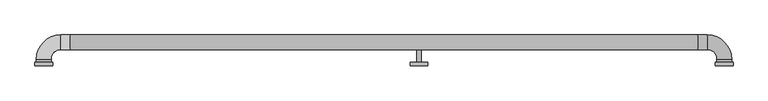
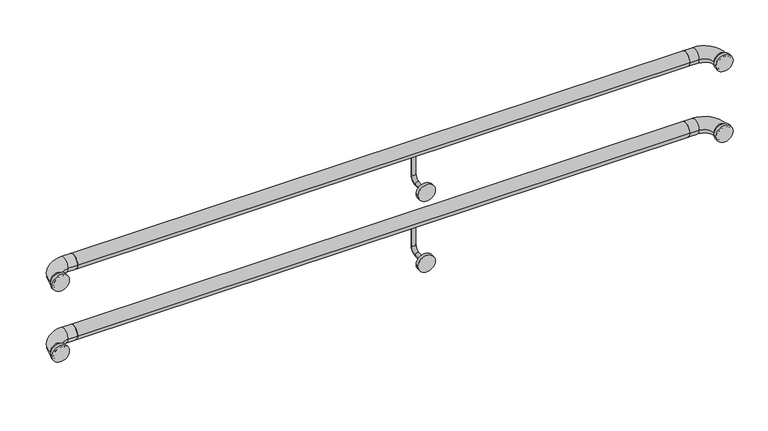
"""IFC4 building model written with IfcOpenShell, lengths in millimetres: railing geometry."""

from ifc_helpers import new_model, si_unit, point, frame, frame_2d, origin, place, context, project, spatial, circle_curve, ellipse_curve, trimmed, segment, composite_curve, outline, extrude, source, transform, mapped, element, save
from ifc_brep_helpers import plane_surface, cylinder_surface, revolved_surface, advanced_brep


def railing_3e29a62d(model_context):
    return source(origin(), model_context, "Body", "SolidModel", [
        extrude(outline(composite_curve([segment(trimmed(circle_curve(frame_2d((33728.1400611, 899.0)), 21.0), [point((33749.1400611, 899.0))], [point((33707.1400611, 899.0))], False, "CARTESIAN"), True, "CONTINUOUS"), segment(trimmed(circle_curve(frame_2d((33728.1400611, 899.0)), 21.0), [point((33707.1400611, 899.0))], [point((33749.1400611, 899.0))], False, "CARTESIAN"), True, "CONTINUOUS")], self_intersect=False)), frame((9766.6129185, 0.0, 0.0), z_axis=(1.0, 0.0, 0.0), x_axis=(0.0, 1.0, 0.0)), (0.0, 0.0, 1.0), 1800.0),
        extrude(outline(composite_curve([segment(trimmed(circle_curve(frame_2d((33728.1400611, 679.0)), 21.0), [point((33749.1400611, 679.0))], [point((33707.1400611, 679.0))], False, "CARTESIAN"), True, "CONTINUOUS"), segment(trimmed(circle_curve(frame_2d((33728.1400611, 679.0)), 21.0), [point((33707.1400611, 679.0))], [point((33749.1400611, 679.0))], False, "CARTESIAN"), True, "CONTINUOUS")], self_intersect=False)), frame((9766.6129185, 0.0, 0.0), z_axis=(1.0, 0.0, 0.0), x_axis=(0.0, 1.0, 0.0)), (0.0, 0.0, 1.0), 1800.0),
        extrude(outline(composite_curve([segment(trimmed(circle_curve(frame_2d((582.0, 10766.6129185)), 25.4), [point((582.0, 10792.0129185))], [point((582.0, 10741.2129185))], False, "CARTESIAN"), True, "CONTINUOUS"), segment(trimmed(circle_curve(frame_2d((582.0, 10766.6129185)), 25.4), [point((582.0, 10741.2129185))], [point((582.0, 10792.0129185))], False, "CARTESIAN"), True, "CONTINUOUS")], self_intersect=False)), frame((0.0, 33661.1900611, 0.0), z_axis=(0.0, 1.0, 0.0), x_axis=(0.0, 0.0, 1.0)), (0.0, 0.0, 1.0), 9.525),
        extrude(outline(composite_curve([segment(trimmed(circle_curve(frame_2d((802.0, 10766.6129185)), 25.4), [point((802.0, 10792.0129185))], [point((802.0, 10741.2129185))], False, "CARTESIAN"), True, "CONTINUOUS"), segment(trimmed(circle_curve(frame_2d((802.0, 10766.6129185)), 25.4), [point((802.0, 10741.2129185))], [point((802.0, 10792.0129185))], False, "CARTESIAN"), True, "CONTINUOUS")], self_intersect=False)), frame((0.0, 33661.1900611, 0.0), z_axis=(0.0, 1.0, 0.0), x_axis=(0.0, 0.0, 1.0)), (0.0, 0.0, 1.0), 9.525),
        advanced_brep(
        [(10760.2629185, 33728.1900611, 658.0), (10772.9629185, 33728.1900611, 658.0), (10760.2629185, 33728.1900611, 601.05), (10772.9629185, 33728.1900611, 601.05), (10772.9629185, 33709.1400611, 582.0), (10760.2629185, 33709.1400611, 582.0), (10760.2629185, 33670.7150611, 582.0), (10772.9629185, 33670.7150611, 582.0)],
        [
            (0, 1, circle_curve(frame((10766.6129185, 33728.1900611, 658.0), z_axis=(0.0, 0.0, 1.0), x_axis=(1.0, 0.0, 0.0)), 6.35)),
            (1, 0, circle_curve(frame((10766.6129185, 33728.1900611, 658.0), z_axis=(0.0, 0.0, 1.0), x_axis=(1.0, 0.0, 0.0)), 6.35)),
            (0, 2),
            (2, 3, circle_curve(frame((10766.6129185, 33728.1900611, 601.05), z_axis=(0.0, 0.0, 1.0), x_axis=(1.0, 0.0, 0.0)), 6.35)),
            (3, 1),
            (3, 2, circle_curve(frame((10766.6129185, 33728.1900611, 601.05), z_axis=(0.0, 0.0, 1.0), x_axis=(1.0, 0.0, 0.0)), 6.35)),
            (4, 3, circle_curve(frame((10772.9629185, 33709.1400611, 601.05), z_axis=(1.0, 0.0, 0.0), x_axis=(0.0, 1.0, 0.0)), 19.05)),
            (2, 5, circle_curve(frame((10760.2629185, 33709.1400611, 601.05), z_axis=(-1.0, 0.0, 0.0), x_axis=(0.0, 1.0, 0.0)), 19.05)),
            (5, 4, circle_curve(frame((10766.6129185, 33709.1400611, 582.0), z_axis=(0.0, 1.0, 0.0), x_axis=(1.0, 0.0, 0.0)), 6.35)),
            (4, 5, circle_curve(frame((10766.6129185, 33709.1400611, 582.0), z_axis=(0.0, 1.0, 0.0), x_axis=(1.0, 0.0, 0.0)), 6.35)),
            (6, 7, circle_curve(frame((10766.6129185, 33670.7150611, 582.0), z_axis=(0.0, -1.0, 0.0), x_axis=(1.0, 0.0, 0.0)), 6.35)),
            (7, 6, circle_curve(frame((10766.6129185, 33670.7150611, 582.0), z_axis=(0.0, -1.0, 0.0), x_axis=(1.0, 0.0, 0.0)), 6.35)),
            (5, 6),
            (7, 4),
        ],
        [
            plane_surface(frame((10772.9629185, 33728.1900611, 658.0), z_axis=(0.0, 0.0, 1.0), x_axis=(0.0, -1.0, 0.0))),
            cylinder_surface(frame((10766.6129185, 33728.1900611, 658.0), z_axis=(0.0, 0.0, 1.0), x_axis=(1.0, 0.0, 0.0)), 6.35),
            revolved_surface(trimmed(ellipse_curve(frame((10766.6129185, 33728.1900611, 601.05), z_axis=(0.0, 0.0, 1.0), x_axis=(1.0, 0.0, 0.0)), 6.35, 6.35), [point((10760.2629185, 33728.1900611, 601.05))], [point((10772.9629185, 33728.1900611, 601.05))], True, "CARTESIAN"), (10766.6129185, 33709.1400611, 601.05), (-1.0, 0.0, 0.0)),
            revolved_surface(trimmed(ellipse_curve(frame((10766.6129185, 33728.1900611, 601.05), z_axis=(0.0, 0.0, 1.0), x_axis=(1.0, 0.0, 0.0)), 6.35, 6.35), [point((10772.9629185, 33728.1900611, 601.05))], [point((10760.2629185, 33728.1900611, 601.05))], True, "CARTESIAN"), (10766.6129185, 33709.1400611, 601.05), (-1.0, 0.0, 0.0)),
            plane_surface(frame((10766.6129185, 33670.7150611, 575.65), z_axis=(0.0, -1.0, 0.0), x_axis=(1.0, 0.0, 0.0))),
            cylinder_surface(frame((10766.6129185, 33709.1400611, 582.0), z_axis=(0.0, 1.0, 0.0), x_axis=(1.0, 0.0, 0.0)), 6.35),
        ],
        [
            (0, [[1, 2]]),
            (1, [[-1, 3, 4, 5]]),
            (1, [[-2, -5, 6, -3]]),
            (2, [[7, -4, 8, 9]]),
            (3, [[-8, -6, -7, 10]]),
            (4, [[11, 12]]),
            (5, [[-9, 13, -12, 14]]),
            (5, [[-10, -14, -11, -13]]),
        ],
    ),
        advanced_brep(
        [(10760.2629185, 33728.1900611, 878.0), (10772.9629185, 33728.1900611, 878.0), (10760.2629185, 33728.1900611, 821.05), (10772.9629185, 33728.1900611, 821.05), (10772.9629185, 33709.1400611, 802.0), (10760.2629185, 33709.1400611, 802.0), (10760.2629185, 33670.7150611, 802.0), (10772.9629185, 33670.7150611, 802.0)],
        [
            (0, 1, circle_curve(frame((10766.6129185, 33728.1900611, 878.0), z_axis=(0.0, 0.0, 1.0), x_axis=(1.0, 0.0, 0.0)), 6.35)),
            (1, 0, circle_curve(frame((10766.6129185, 33728.1900611, 878.0), z_axis=(0.0, 0.0, 1.0), x_axis=(1.0, 0.0, 0.0)), 6.35)),
            (0, 2),
            (2, 3, circle_curve(frame((10766.6129185, 33728.1900611, 821.05), z_axis=(0.0, 0.0, 1.0), x_axis=(1.0, 0.0, 0.0)), 6.35)),
            (3, 1),
            (3, 2, circle_curve(frame((10766.6129185, 33728.1900611, 821.05), z_axis=(0.0, 0.0, 1.0), x_axis=(1.0, 0.0, 0.0)), 6.35)),
            (4, 3, circle_curve(frame((10772.9629185, 33709.1400611, 821.05), z_axis=(1.0, 0.0, 0.0), x_axis=(0.0, 1.0, 0.0)), 19.05)),
            (2, 5, circle_curve(frame((10760.2629185, 33709.1400611, 821.05), z_axis=(-1.0, 0.0, 0.0), x_axis=(0.0, 1.0, 0.0)), 19.05)),
            (5, 4, circle_curve(frame((10766.6129185, 33709.1400611, 802.0), z_axis=(0.0, 1.0, 0.0), x_axis=(1.0, 0.0, 0.0)), 6.35)),
            (4, 5, circle_curve(frame((10766.6129185, 33709.1400611, 802.0), z_axis=(0.0, 1.0, 0.0), x_axis=(1.0, 0.0, 0.0)), 6.35)),
            (6, 7, circle_curve(frame((10766.6129185, 33670.7150611, 802.0), z_axis=(0.0, -1.0, 0.0), x_axis=(1.0, 0.0, 0.0)), 6.35)),
            (7, 6, circle_curve(frame((10766.6129185, 33670.7150611, 802.0), z_axis=(0.0, -1.0, 0.0), x_axis=(1.0, 0.0, 0.0)), 6.35)),
            (5, 6),
            (7, 4),
        ],
        [
            plane_surface(frame((10772.9629185, 33728.1900611, 878.0), z_axis=(0.0, 0.0, 1.0), x_axis=(0.0, -1.0, 0.0))),
            cylinder_surface(frame((10766.6129185, 33728.1900611, 878.0), z_axis=(0.0, 0.0, 1.0), x_axis=(1.0, 0.0, 0.0)), 6.35),
            revolved_surface(trimmed(ellipse_curve(frame((10766.6129185, 33728.1900611, 821.05), z_axis=(0.0, 0.0, 1.0), x_axis=(1.0, 0.0, 0.0)), 6.35, 6.35), [point((10760.2629185, 33728.1900611, 821.05))], [point((10772.9629185, 33728.1900611, 821.05))], True, "CARTESIAN"), (10766.6129185, 33709.1400611, 821.05), (-1.0, 0.0, 0.0)),
            revolved_surface(trimmed(ellipse_curve(frame((10766.6129185, 33728.1900611, 821.05), z_axis=(0.0, 0.0, 1.0), x_axis=(1.0, 0.0, 0.0)), 6.35, 6.35), [point((10772.9629185, 33728.1900611, 821.05))], [point((10760.2629185, 33728.1900611, 821.05))], True, "CARTESIAN"), (10766.6129185, 33709.1400611, 821.05), (-1.0, 0.0, 0.0)),
            plane_surface(frame((10766.6129185, 33670.7150611, 795.65), z_axis=(0.0, -1.0, 0.0), x_axis=(1.0, 0.0, 0.0))),
            cylinder_surface(frame((10766.6129185, 33709.1400611, 802.0), z_axis=(0.0, 1.0, 0.0), x_axis=(1.0, 0.0, 0.0)), 6.35),
        ],
        [
            (0, [[1, 2]]),
            (1, [[-1, 3, 4, 5]]),
            (1, [[-2, -5, 6, -3]]),
            (2, [[7, -4, 8, 9]]),
            (3, [[-8, -6, -7, 10]]),
            (4, [[11, 12]]),
            (5, [[-9, 13, -12, 14]]),
            (5, [[-10, -14, -11, -13]]),
        ],
    ),
        extrude(outline(composite_curve([segment(trimmed(circle_curve(frame_2d((679.1, 11642.6129185)), 25.4), [point((679.1, 11668.0129185))], [point((679.1, 11617.2129185))], False, "CARTESIAN"), True, "CONTINUOUS"), segment(trimmed(circle_curve(frame_2d((679.1, 11642.6129185)), 25.4), [point((679.1, 11617.2129185))], [point((679.1, 11668.0129185))], False, "CARTESIAN"), True, "CONTINUOUS")], self_intersect=False)), frame((0.0, 33661.1900611, 0.0), z_axis=(0.0, 1.0, 0.0), x_axis=(0.0, 0.0, 1.0)), (0.0, 0.0, 1.0), 9.525),
        extrude(outline(composite_curve([segment(trimmed(circle_curve(frame_2d((899.1, 11642.6129185)), 25.4), [point((899.1, 11668.0129185))], [point((899.1, 11617.2129185))], False, "CARTESIAN"), True, "CONTINUOUS"), segment(trimmed(circle_curve(frame_2d((899.1, 11642.6129185)), 25.4), [point((899.1, 11617.2129185))], [point((899.1, 11668.0129185))], False, "CARTESIAN"), True, "CONTINUOUS")], self_intersect=False)), frame((0.0, 33661.1900611, 0.0), z_axis=(0.0, 1.0, 0.0), x_axis=(0.0, 0.0, 1.0)), (0.0, 0.0, 1.0), 9.525),
        advanced_brep(
        [(11566.6129185, 33707.1900611, 679.1), (11566.6129185, 33749.1900611, 679.1), (11594.1129185, 33707.1900611, 679.1), (11594.1129185, 33749.1900611, 679.1), (11663.6129185, 33679.6900611, 679.1), (11621.6129185, 33679.6900611, 679.1), (11621.6129185, 33661.1900611, 679.1), (11663.6129185, 33661.1900611, 679.1)],
        [
            (0, 1, circle_curve(frame((11566.6129185, 33728.1900611, 679.1), z_axis=(-1.0, 0.0, 0.0), x_axis=(0.0, 1.0, 0.0)), 21.0)),
            (1, 0, circle_curve(frame((11566.6129185, 33728.1900611, 679.1), z_axis=(-1.0, 0.0, 0.0), x_axis=(0.0, 1.0, 0.0)), 21.0)),
            (0, 2),
            (2, 3, circle_curve(frame((11594.1129185, 33728.1900611, 679.1), z_axis=(-1.0, 0.0, 0.0), x_axis=(0.0, 1.0, 0.0)), 21.0)),
            (3, 1),
            (3, 2, circle_curve(frame((11594.1129185, 33728.1900611, 679.1), z_axis=(-1.0, 0.0, 0.0), x_axis=(0.0, 1.0, 0.0)), 21.0)),
            (4, 3, circle_curve(frame((11594.1129185, 33679.6900611, 679.1), z_axis=(0.0, 0.0, 1.0), x_axis=(0.0, 1.0, 0.0)), 69.5)),
            (2, 5, circle_curve(frame((11594.1129185, 33679.6900611, 679.1), z_axis=(0.0, 0.0, -1.0), x_axis=(0.0, 1.0, 0.0)), 27.5)),
            (5, 4, circle_curve(frame((11642.6129185, 33679.6900611, 679.1), z_axis=(0.0, 1.0, 0.0), x_axis=(1.0, 0.0, 0.0)), 21.0)),
            (4, 5, circle_curve(frame((11642.6129185, 33679.6900611, 679.1), z_axis=(0.0, 1.0, 0.0), x_axis=(1.0, 0.0, 0.0)), 21.0)),
            (6, 7, circle_curve(frame((11642.6129185, 33661.1900611, 679.1), z_axis=(0.0, -1.0, 0.0), x_axis=(1.0, 0.0, 0.0)), 21.0)),
            (7, 6, circle_curve(frame((11642.6129185, 33661.1900611, 679.1), z_axis=(0.0, -1.0, 0.0), x_axis=(1.0, 0.0, 0.0)), 21.0)),
            (5, 6),
            (7, 4),
        ],
        [
            plane_surface(frame((11566.6129185, 33728.1900611, 679.1), z_axis=(-1.0, 0.0, 0.0), x_axis=(0.0, 0.0, 1.0))),
            cylinder_surface(frame((11566.6129185, 33728.1900611, 679.1), z_axis=(-1.0, 0.0, 0.0), x_axis=(0.0, 1.0, 0.0)), 21.0),
            revolved_surface(trimmed(ellipse_curve(frame((11594.1129185, 33728.1900611, 679.1), z_axis=(-1.0, 0.0, 0.0), x_axis=(0.0, 1.0, 0.0)), 21.0, 21.0), [point((11594.1129185, 33707.1900611, 679.1))], [point((11594.1129185, 33749.1900611, 679.1))], True, "CARTESIAN"), (11594.1129185, 33679.6900611, 679.1), (0.0, 0.0, -1.0)),
            revolved_surface(trimmed(ellipse_curve(frame((11594.1129185, 33728.1900611, 679.1), z_axis=(-1.0, 0.0, 0.0), x_axis=(0.0, 1.0, 0.0)), 21.0, 21.0), [point((11594.1129185, 33749.1900611, 679.1))], [point((11594.1129185, 33707.1900611, 679.1))], True, "CARTESIAN"), (11594.1129185, 33679.6900611, 679.1), (0.0, 0.0, -1.0)),
            plane_surface(frame((11642.6129185, 33661.1900611, 679.1), z_axis=(0.0, -1.0, 0.0), x_axis=(0.0, 0.0, 1.0))),
            cylinder_surface(frame((11642.6129185, 33679.6900611, 679.1), z_axis=(0.0, 1.0, 0.0), x_axis=(1.0, 0.0, 0.0)), 21.0),
        ],
        [
            (0, [[1, 2]]),
            (1, [[-1, 3, 4, 5]]),
            (1, [[-2, -5, 6, -3]]),
            (2, [[7, -4, 8, 9]]),
            (3, [[-8, -6, -7, 10]]),
            (4, [[11, 12]]),
            (5, [[-9, 13, -12, 14]]),
            (5, [[-10, -14, -11, -13]]),
        ],
    ),
        advanced_brep(
        [(11566.6129185, 33707.1900611, 899.1), (11566.6129185, 33749.1900611, 899.1), (11594.1129185, 33707.1900611, 899.1), (11594.1129185, 33749.1900611, 899.1), (11663.6129185, 33679.6900611, 899.1), (11621.6129185, 33679.6900611, 899.1), (11621.6129185, 33661.1900611, 899.1), (11663.6129185, 33661.1900611, 899.1)],
        [
            (0, 1, circle_curve(frame((11566.6129185, 33728.1900611, 899.1), z_axis=(-1.0, 0.0, 0.0), x_axis=(0.0, 1.0, 0.0)), 21.0)),
            (1, 0, circle_curve(frame((11566.6129185, 33728.1900611, 899.1), z_axis=(-1.0, 0.0, 0.0), x_axis=(0.0, 1.0, 0.0)), 21.0)),
            (0, 2),
            (2, 3, circle_curve(frame((11594.1129185, 33728.1900611, 899.1), z_axis=(-1.0, 0.0, 0.0), x_axis=(0.0, 1.0, 0.0)), 21.0)),
            (3, 1),
            (3, 2, circle_curve(frame((11594.1129185, 33728.1900611, 899.1), z_axis=(-1.0, 0.0, 0.0), x_axis=(0.0, 1.0, 0.0)), 21.0)),
            (4, 3, circle_curve(frame((11594.1129185, 33679.6900611, 899.1), z_axis=(0.0, 0.0, 1.0), x_axis=(0.0, 1.0, 0.0)), 69.5)),
            (2, 5, circle_curve(frame((11594.1129185, 33679.6900611, 899.1), z_axis=(0.0, 0.0, -1.0), x_axis=(0.0, 1.0, 0.0)), 27.5)),
            (5, 4, circle_curve(frame((11642.6129185, 33679.6900611, 899.1), z_axis=(0.0, 1.0, 0.0), x_axis=(1.0, 0.0, 0.0)), 21.0)),
            (4, 5, circle_curve(frame((11642.6129185, 33679.6900611, 899.1), z_axis=(0.0, 1.0, 0.0), x_axis=(1.0, 0.0, 0.0)), 21.0)),
            (6, 7, circle_curve(frame((11642.6129185, 33661.1900611, 899.1), z_axis=(0.0, -1.0, 0.0), x_axis=(1.0, 0.0, 0.0)), 21.0)),
            (7, 6, circle_curve(frame((11642.6129185, 33661.1900611, 899.1), z_axis=(0.0, -1.0, 0.0), x_axis=(1.0, 0.0, 0.0)), 21.0)),
            (5, 6),
            (7, 4),
        ],
        [
            plane_surface(frame((11566.6129185, 33728.1900611, 899.1), z_axis=(-1.0, 0.0, 0.0), x_axis=(0.0, 0.0, 1.0))),
            cylinder_surface(frame((11566.6129185, 33728.1900611, 899.1), z_axis=(-1.0, 0.0, 0.0), x_axis=(0.0, 1.0, 0.0)), 21.0),
            revolved_surface(trimmed(ellipse_curve(frame((11594.1129185, 33728.1900611, 899.1), z_axis=(-1.0, 0.0, 0.0), x_axis=(0.0, 1.0, 0.0)), 21.0, 21.0), [point((11594.1129185, 33707.1900611, 899.1))], [point((11594.1129185, 33749.1900611, 899.1))], True, "CARTESIAN"), (11594.1129185, 33679.6900611, 899.1), (0.0, 0.0, -1.0)),
            revolved_surface(trimmed(ellipse_curve(frame((11594.1129185, 33728.1900611, 899.1), z_axis=(-1.0, 0.0, 0.0), x_axis=(0.0, 1.0, 0.0)), 21.0, 21.0), [point((11594.1129185, 33749.1900611, 899.1))], [point((11594.1129185, 33707.1900611, 899.1))], True, "CARTESIAN"), (11594.1129185, 33679.6900611, 899.1), (0.0, 0.0, -1.0)),
            plane_surface(frame((11642.6129185, 33661.1900611, 899.1), z_axis=(0.0, -1.0, 0.0), x_axis=(0.0, 0.0, 1.0))),
            cylinder_surface(frame((11642.6129185, 33679.6900611, 899.1), z_axis=(0.0, 1.0, 0.0), x_axis=(1.0, 0.0, 0.0)), 21.0),
        ],
        [
            (0, [[1, 2]]),
            (1, [[-1, 3, 4, 5]]),
            (1, [[-2, -5, 6, -3]]),
            (2, [[7, -4, 8, 9]]),
            (3, [[-8, -6, -7, 10]]),
            (4, [[11, 12]]),
            (5, [[-9, 13, -12, 14]]),
            (5, [[-10, -14, -11, -13]]),
        ],
    ),
        extrude(outline(composite_curve([segment(trimmed(circle_curve(frame_2d((679.1, 9690.6129185)), 25.4), [point((679.1, 9716.0129185))], [point((679.1, 9665.2129185))], False, "CARTESIAN"), True, "CONTINUOUS"), segment(trimmed(circle_curve(frame_2d((679.1, 9690.6129185)), 25.4), [point((679.1, 9665.2129185))], [point((679.1, 9716.0129185))], False, "CARTESIAN"), True, "CONTINUOUS")], self_intersect=False)), frame((0.0, 33661.1900611, 0.0), z_axis=(0.0, 1.0, 0.0), x_axis=(0.0, 0.0, 1.0)), (0.0, 0.0, 1.0), 9.525),
        extrude(outline(composite_curve([segment(trimmed(circle_curve(frame_2d((899.1, 9690.6129185)), 25.4), [point((899.1, 9716.0129185))], [point((899.1, 9665.2129185))], False, "CARTESIAN"), True, "CONTINUOUS"), segment(trimmed(circle_curve(frame_2d((899.1, 9690.6129185)), 25.4), [point((899.1, 9665.2129185))], [point((899.1, 9716.0129185))], False, "CARTESIAN"), True, "CONTINUOUS")], self_intersect=False)), frame((0.0, 33661.1900611, 0.0), z_axis=(0.0, 1.0, 0.0), x_axis=(0.0, 0.0, 1.0)), (0.0, 0.0, 1.0), 9.525),
        advanced_brep(
        [(9766.6129185, 33749.1900611, 679.1), (9766.6129185, 33707.1900611, 679.1), (9739.1129185, 33707.1900611, 679.1), (9739.1129185, 33749.1900611, 679.1), (9669.6129185, 33679.6900611, 679.1), (9711.6129185, 33679.6900611, 679.1), (9711.6129185, 33661.1900611, 679.1), (9669.6129185, 33661.1900611, 679.1)],
        [
            (0, 1, circle_curve(frame((9766.6129185, 33728.1900611, 679.1), z_axis=(1.0, 0.0, 0.0), x_axis=(0.0, -1.0, 0.0)), 21.0)),
            (1, 0, circle_curve(frame((9766.6129185, 33728.1900611, 679.1), z_axis=(1.0, 0.0, 0.0), x_axis=(0.0, -1.0, 0.0)), 21.0)),
            (1, 2),
            (2, 3, circle_curve(frame((9739.1129185, 33728.1900611, 679.1), z_axis=(1.0, 0.0, 0.0), x_axis=(0.0, -1.0, 0.0)), 21.0)),
            (3, 0),
            (3, 2, circle_curve(frame((9739.1129185, 33728.1900611, 679.1), z_axis=(1.0, 0.0, 0.0), x_axis=(0.0, -1.0, 0.0)), 21.0)),
            (4, 3, circle_curve(frame((9739.1129185, 33679.6900611, 679.1), z_axis=(0.0, 0.0, -1.0), x_axis=(0.0, 1.0, 0.0)), 69.5)),
            (2, 5, circle_curve(frame((9739.1129185, 33679.6900611, 679.1), z_axis=(0.0, 0.0, 1.0), x_axis=(0.0, 1.0, 0.0)), 27.5)),
            (5, 4, circle_curve(frame((9690.6129185, 33679.6900611, 679.1), z_axis=(0.0, 1.0, 0.0), x_axis=(1.0, 0.0, 0.0)), 21.0)),
            (4, 5, circle_curve(frame((9690.6129185, 33679.6900611, 679.1), z_axis=(0.0, 1.0, 0.0), x_axis=(1.0, 0.0, 0.0)), 21.0)),
            (5, 6),
            (6, 7, circle_curve(frame((9690.6129185, 33661.1900611, 679.1), z_axis=(0.0, 1.0, 0.0), x_axis=(1.0, 0.0, 0.0)), 21.0)),
            (7, 4),
            (7, 6, circle_curve(frame((9690.6129185, 33661.1900611, 679.1), z_axis=(0.0, 1.0, 0.0), x_axis=(1.0, 0.0, 0.0)), 21.0)),
        ],
        [
            plane_surface(frame((9766.6129185, 33728.1900611, 679.1), z_axis=(1.0, 0.0, 0.0), x_axis=(0.0, 0.0, 1.0))),
            cylinder_surface(frame((9766.6129185, 33728.1900611, 679.1), z_axis=(1.0, 0.0, 0.0), x_axis=(0.0, -1.0, 0.0)), 21.0),
            revolved_surface(trimmed(ellipse_curve(frame((9739.1129185, 33728.1900611, 679.1), z_axis=(1.0, 0.0, 0.0), x_axis=(0.0, -1.0, 0.0)), 21.0, 21.0), [point((9739.1129185, 33707.1900611, 679.1))], [point((9739.1129185, 33749.1900611, 679.1))], True, "CARTESIAN"), (9739.1129185, 33679.6900611, 679.1), (0.0, 0.0, 1.0)),
            revolved_surface(trimmed(ellipse_curve(frame((9739.1129185, 33728.1900611, 679.1), z_axis=(1.0, 0.0, 0.0), x_axis=(0.0, -1.0, 0.0)), 21.0, 21.0), [point((9739.1129185, 33749.1900611, 679.1))], [point((9739.1129185, 33707.1900611, 679.1))], True, "CARTESIAN"), (9739.1129185, 33679.6900611, 679.1), (0.0, 0.0, 1.0)),
            cylinder_surface(frame((9690.6129185, 33679.6900611, 679.1), z_axis=(0.0, 1.0, 0.0), x_axis=(1.0, 0.0, 0.0)), 21.0),
            plane_surface(frame((9690.6129185, 33661.1900611, 679.1), z_axis=(0.0, -1.0, 0.0), x_axis=(0.0, 0.0, 1.0))),
        ],
        [
            (0, [[1, 2]]),
            (1, [[-2, 3, 4, 5]]),
            (1, [[-1, -5, 6, -3]]),
            (2, [[7, -4, 8, 9]]),
            (3, [[-8, -6, -7, 10]]),
            (4, [[-9, 11, 12, 13]]),
            (4, [[-10, -13, 14, -11]]),
            (5, [[-12, -14]]),
        ],
    ),
        advanced_brep(
        [(9766.6129185, 33749.1900611, 899.1), (9766.6129185, 33707.1900611, 899.1), (9739.1129185, 33707.1900611, 899.1), (9739.1129185, 33749.1900611, 899.1), (9669.6129185, 33679.6900611, 899.1), (9711.6129185, 33679.6900611, 899.1), (9669.6129185, 33661.1900611, 899.1), (9711.6129185, 33661.1900611, 899.1)],
        [
            (0, 1, circle_curve(frame((9766.6129185, 33728.1900611, 899.1), z_axis=(1.0, 0.0, 0.0), x_axis=(0.0, -1.0, 0.0)), 21.0)),
            (1, 0, circle_curve(frame((9766.6129185, 33728.1900611, 899.1), z_axis=(1.0, 0.0, 0.0), x_axis=(0.0, -1.0, 0.0)), 21.0)),
            (1, 2),
            (2, 3, circle_curve(frame((9739.1129185, 33728.1900611, 899.1), z_axis=(1.0, 0.0, 0.0), x_axis=(0.0, -1.0, 0.0)), 21.0)),
            (3, 0),
            (3, 2, circle_curve(frame((9739.1129185, 33728.1900611, 899.1), z_axis=(1.0, 0.0, 0.0), x_axis=(0.0, -1.0, 0.0)), 21.0)),
            (4, 3, circle_curve(frame((9739.1129185, 33679.6900611, 899.1), z_axis=(0.0, 0.0, -1.0), x_axis=(0.0, 1.0, 0.0)), 69.5)),
            (2, 5, circle_curve(frame((9739.1129185, 33679.6900611, 899.1), z_axis=(0.0, 0.0, 1.0), x_axis=(0.0, 1.0, 0.0)), 27.5)),
            (5, 4, circle_curve(frame((9690.6129185, 33679.6900611, 899.1), z_axis=(0.0, 1.0, 0.0), x_axis=(1.0, 0.0, 0.0)), 21.0)),
            (4, 5, circle_curve(frame((9690.6129185, 33679.6900611, 899.1), z_axis=(0.0, 1.0, 0.0), x_axis=(1.0, 0.0, 0.0)), 21.0)),
            (6, 7, circle_curve(frame((9690.6129185, 33661.1900611, 899.1), z_axis=(0.0, -1.0, 0.0), x_axis=(1.0, 0.0, 0.0)), 21.0)),
            (7, 6, circle_curve(frame((9690.6129185, 33661.1900611, 899.1), z_axis=(0.0, -1.0, 0.0), x_axis=(1.0, 0.0, 0.0)), 21.0)),
            (5, 7),
            (6, 4),
        ],
        [
            plane_surface(frame((9766.6129185, 33728.1900611, 899.1), z_axis=(1.0, 0.0, 0.0), x_axis=(0.0, 0.0, 1.0))),
            cylinder_surface(frame((9766.6129185, 33728.1900611, 899.1), z_axis=(1.0, 0.0, 0.0), x_axis=(0.0, -1.0, 0.0)), 21.0),
            revolved_surface(trimmed(ellipse_curve(frame((9739.1129185, 33728.1900611, 899.1), z_axis=(1.0, 0.0, 0.0), x_axis=(0.0, -1.0, 0.0)), 21.0, 21.0), [point((9739.1129185, 33707.1900611, 899.1))], [point((9739.1129185, 33749.1900611, 899.1))], True, "CARTESIAN"), (9739.1129185, 33679.6900611, 899.1), (0.0, 0.0, 1.0)),
            revolved_surface(trimmed(ellipse_curve(frame((9739.1129185, 33728.1900611, 899.1), z_axis=(1.0, 0.0, 0.0), x_axis=(0.0, -1.0, 0.0)), 21.0, 21.0), [point((9739.1129185, 33749.1900611, 899.1))], [point((9739.1129185, 33707.1900611, 899.1))], True, "CARTESIAN"), (9739.1129185, 33679.6900611, 899.1), (0.0, 0.0, 1.0)),
            plane_surface(frame((9690.6129185, 33661.1900611, 899.1), z_axis=(0.0, -1.0, 0.0), x_axis=(0.0, 0.0, 1.0))),
            cylinder_surface(frame((9690.6129185, 33679.6900611, 899.1), z_axis=(0.0, 1.0, 0.0), x_axis=(1.0, 0.0, 0.0)), 21.0),
        ],
        [
            (0, [[1, 2]]),
            (1, [[-2, 3, 4, 5]]),
            (1, [[-1, -5, 6, -3]]),
            (2, [[7, -4, 8, 9]]),
            (3, [[-8, -6, -7, 10]]),
            (4, [[11, 12]]),
            (5, [[-9, 13, -11, 14]]),
            (5, [[-10, -14, -12, -13]]),
        ],
    ),
    ])


if __name__ == "__main__":
    model = new_model("IFC4")
    model_context = context("Model", 3, world=origin())
    ifc_project = project(units=[si_unit("LENGTHUNIT", "METRE", prefix="MILLI")], contexts=[model_context])
    site = spatial("IfcSite", under=ifc_project)
    building = spatial("IfcBuilding", under=site)
    placement = place(None, origin())
    railing_shape = railing_3e29a62d(model_context)
    element("IfcRailing", 1, at=placement, inside=building, context=model_context, shape_type="MappedRepresentation", body=[
        mapped(railing_shape, transform((0.0, 0.0, 0.0), x_axis=(1.0, 0.0, 0.0), y_axis=(0.0, 1.0, 0.0), z_axis=(0.0, 0.0, 1.0))),
    ])
    save(model, "model.ifc")

# Revit data of these elements
# Element 1 (IfcRailing)
#   Materials on its faces: "Ferro - Pintura Esmalte"
# Materials
#   "Ferro - Pintura Esmalte": class "Pintura", colour RGB 255 255 255, transparency 0, Cost = 0
